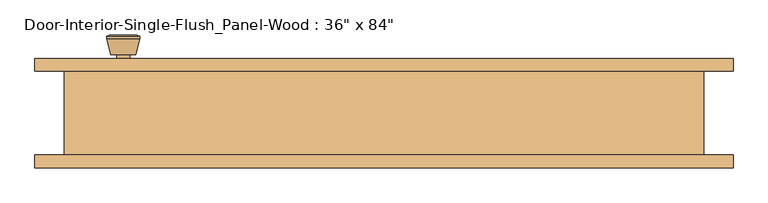
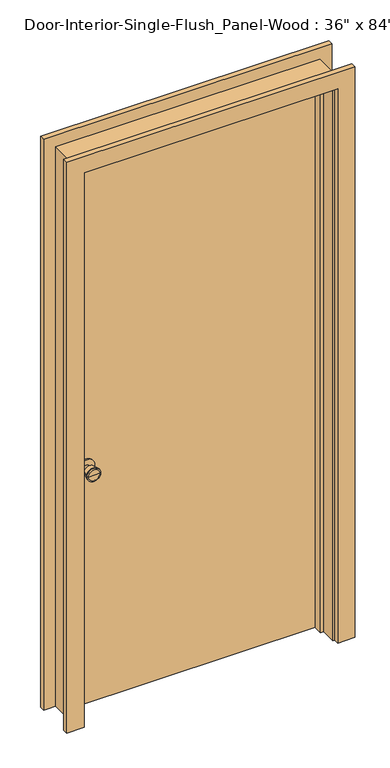
"""IFC4 building model written with IfcOpenShell, lengths in millimetres: door geometry."""

from ifc_helpers import new_model, si_unit, point, frame, frame_2d, origin, origin_with_axes, place, context, project, spatial, polyline, circle_curve, trimmed, segment, composite_curve, outline, extrude, faceted_brep, source, transform, mapped, element, save
from ifc_brep_helpers import plane_surface, cylinder_surface, revolved_surface, advanced_brep


def door_77100466(model_context):
    return source(origin(), model_context, "Body", "SolidModel", [
        advanced_brep(
        [(-393.7, 19.4, 914.4), (-383.7, 19.4, 914.4), (-403.7, 19.4, 914.4), (-373.2241324, -29.6, 914.4), (-393.7, -29.6, 914.4), (-414.1758676, -29.6, 914.4), (-368.7, -27.7721319, 914.4), (-418.7, -27.7721319, 914.4), (-368.7, -24.3084537, 914.4), (-418.7, -24.3084537, 914.4), (-375.063764, 0.4, 914.4), (-412.336236, 0.4, 914.4), (-383.7, 0.4, 914.4), (-403.7, 0.4, 914.4)],
        [
            (0, 1),
            (1, 2, circle_curve(frame((-393.7, 19.4, 914.4), z_axis=(0.0, 1.0, 0.0), x_axis=(-1.0, 0.0, 0.0)), 10.0)),
            (2, 0),
            (2, 1, circle_curve(frame((-393.7, 19.4, 914.4), z_axis=(0.0, 1.0, 0.0), x_axis=(-1.0, 0.0, 0.0)), 10.0)),
            (3, 4),
            (4, 5),
            (5, 3, circle_curve(frame((-393.7, -29.6, 914.4), z_axis=(0.0, -1.0, 0.0), x_axis=(-1.0, 0.0, 0.0)), 20.4758676)),
            (3, 5, circle_curve(frame((-393.7, -29.6, 914.4), z_axis=(0.0, -1.0, 0.0), x_axis=(-1.0, 0.0, 0.0)), 20.4758676)),
            (6, 3),
            (5, 7),
            (7, 6, circle_curve(frame((-393.7, -27.7721319, 914.4), z_axis=(0.0, -1.0, 0.0), x_axis=(-1.0, 0.0, 0.0)), 25.0)),
            (6, 7, circle_curve(frame((-393.7, -27.7721319, 914.4), z_axis=(0.0, -1.0, 0.0), x_axis=(-1.0, 0.0, 0.0)), 25.0)),
            (8, 6),
            (7, 9),
            (9, 8, circle_curve(frame((-393.7, -24.3084537, 914.4), z_axis=(0.0, -1.0, 0.0), x_axis=(-1.0, 0.0, 0.0)), 25.0)),
            (8, 9, circle_curve(frame((-393.7, -24.3084537, 914.4), z_axis=(0.0, -1.0, 0.0), x_axis=(-1.0, 0.0, 0.0)), 25.0)),
            (10, 8),
            (9, 11),
            (11, 10, circle_curve(frame((-393.7, 0.4, 914.4), z_axis=(0.0, -1.0, 0.0), x_axis=(-1.0, 0.0, 0.0)), 18.636236)),
            (10, 11, circle_curve(frame((-393.7, 0.4, 914.4), z_axis=(0.0, -1.0, 0.0), x_axis=(-1.0, 0.0, 0.0)), 18.636236)),
            (12, 10),
            (11, 13),
            (13, 12, circle_curve(frame((-393.7, 0.4, 914.4), z_axis=(0.0, -1.0, 0.0), x_axis=(-1.0, 0.0, 0.0)), 10.0)),
            (12, 13, circle_curve(frame((-393.7, 0.4, 914.4), z_axis=(0.0, -1.0, 0.0), x_axis=(-1.0, 0.0, 0.0)), 10.0)),
            (1, 12),
            (13, 2),
        ],
        [
            plane_surface(frame((-393.7, 19.4, 914.4), z_axis=(0.0, 1.0, 0.0), x_axis=(-1.0, 0.0, 0.0))),
            plane_surface(frame((-393.7, -29.6, 914.4), z_axis=(0.0, -1.0, 0.0), x_axis=(-1.0, 0.0, 0.0))),
            revolved_surface(polyline([(-414.1758676, -29.6, 914.4), (-418.7, -27.7721319, 914.4)]), (-393.7, 19.4, 914.4), (0.0, 1.0, 0.0)),
            cylinder_surface(frame((-393.7, 19.4, 914.4), z_axis=(0.0, 1.0, 0.0), x_axis=(-1.0, 0.0, 0.0)), 25.0),
            revolved_surface(polyline([(-418.7, -24.3084537, 914.4), (-412.336236, 0.4, 914.4)]), (-393.7, 19.4, 914.4), (0.0, 1.0, 0.0)),
            plane_surface(frame((-393.7, 0.4, 914.4), z_axis=(0.0, 1.0, 0.0), x_axis=(-1.0, 0.0, 0.0))),
            cylinder_surface(frame((-393.7, 19.4, 914.4), z_axis=(0.0, 1.0, 0.0), x_axis=(-1.0, 0.0, 0.0)), 10.0),
        ],
        [
            (0, [[1, 2, 3]]),
            (0, [[-3, 4, -1]]),
            (1, [[5, 6, 7]]),
            (1, [[-6, -5, 8]]),
            (2, [[9, -7, 10, 11]]),
            (2, [[-10, -8, -9, 12]]),
            (3, [[13, -11, 14, 15]]),
            (3, [[-14, -12, -13, 16]]),
            (4, [[17, -15, 18, 19]]),
            (4, [[-18, -16, -17, 20]]),
            (5, [[21, -19, 22, 23]]),
            (5, [[-22, -20, -21, 24]]),
            (6, [[25, -23, 26, -2]]),
            (6, [[-26, -24, -25, -4]]),
        ],
    ),
        extrude(outline(composite_curve([segment(trimmed(circle_curve(frame_2d((914.4, -393.7)), 30.0), [point((914.4, -423.7))], [point((914.4, -363.7))], False, "CARTESIAN"), True, "CONTINUOUS"), segment(trimmed(circle_curve(frame_2d((914.4, -393.7)), 30.0), [point((914.4, -363.7))], [point((914.4, -423.7))], False, "CARTESIAN"), True, "CONTINUOUS")], self_intersect=False)), frame((0.0, 19.4, 0.0), z_axis=(0.0, 1.0, 0.0), x_axis=(0.0, 0.0, 1.0)), (0.0, 0.0, 1.0), 6.0),
        advanced_brep(
        [(-393.7, 66.325, 914.4), (-403.7, 66.325, 914.4), (-383.7, 66.325, 914.4), (-373.2241324, 115.325, 914.4), (-414.1758676, 115.325, 914.4), (-393.7, 115.325, 914.4), (-368.7, 113.4971319, 914.4), (-418.7, 113.4971319, 914.4), (-368.7, 110.0334537, 914.4), (-418.7, 110.0334537, 914.4), (-375.063764, 85.325, 914.4), (-412.336236, 85.325, 914.4), (-383.7, 85.325, 914.4), (-403.7, 85.325, 914.4)],
        [
            (0, 1),
            (1, 2, circle_curve(frame((-393.7, 66.325, 914.4), z_axis=(0.0, -1.0, 0.0), x_axis=(-1.0, 0.0, 0.0)), 10.0)),
            (2, 0),
            (2, 1, circle_curve(frame((-393.7, 66.325, 914.4), z_axis=(0.0, -1.0, 0.0), x_axis=(-1.0, 0.0, 0.0)), 10.0)),
            (3, 4, circle_curve(frame((-393.7, 115.325, 914.4), z_axis=(0.0, 1.0, 0.0), x_axis=(-1.0, 0.0, 0.0)), 20.4758676)),
            (4, 5),
            (5, 3),
            (4, 3, circle_curve(frame((-393.7, 115.325, 914.4), z_axis=(0.0, 1.0, 0.0), x_axis=(-1.0, 0.0, 0.0)), 20.4758676)),
            (6, 7, circle_curve(frame((-393.7, 113.4971319, 914.4), z_axis=(0.0, 1.0, 0.0), x_axis=(-1.0, 0.0, 0.0)), 25.0)),
            (7, 4),
            (3, 6),
            (7, 6, circle_curve(frame((-393.7, 113.4971319, 914.4), z_axis=(0.0, 1.0, 0.0), x_axis=(-1.0, 0.0, 0.0)), 25.0)),
            (8, 9, circle_curve(frame((-393.7, 110.0334537, 914.4), z_axis=(0.0, 1.0, 0.0), x_axis=(-1.0, 0.0, 0.0)), 25.0)),
            (9, 7),
            (6, 8),
            (9, 8, circle_curve(frame((-393.7, 110.0334537, 914.4), z_axis=(0.0, 1.0, 0.0), x_axis=(-1.0, 0.0, 0.0)), 25.0)),
            (10, 11, circle_curve(frame((-393.7, 85.325, 914.4), z_axis=(0.0, 1.0, 0.0), x_axis=(-1.0, 0.0, 0.0)), 18.636236)),
            (11, 9),
            (8, 10),
            (11, 10, circle_curve(frame((-393.7, 85.325, 914.4), z_axis=(0.0, 1.0, 0.0), x_axis=(-1.0, 0.0, 0.0)), 18.636236)),
            (12, 13, circle_curve(frame((-393.7, 85.325, 914.4), z_axis=(0.0, 1.0, 0.0), x_axis=(-1.0, 0.0, 0.0)), 10.0)),
            (13, 11),
            (10, 12),
            (13, 12, circle_curve(frame((-393.7, 85.325, 914.4), z_axis=(0.0, 1.0, 0.0), x_axis=(-1.0, 0.0, 0.0)), 10.0)),
            (1, 13),
            (12, 2),
        ],
        [
            plane_surface(frame((-393.7, 66.325, 914.4), z_axis=(0.0, -1.0, 0.0), x_axis=(-1.0, 0.0, 0.0))),
            plane_surface(frame((-393.7, 115.325, 914.4), z_axis=(0.0, 1.0, 0.0), x_axis=(-1.0, 0.0, 0.0))),
            revolved_surface(polyline([(-414.1758676, 115.325, 914.4), (-418.7, 113.4971319, 914.4)]), (-393.7, 66.325, 914.4), (0.0, -1.0, 0.0)),
            cylinder_surface(frame((-393.7, 66.325, 914.4), z_axis=(0.0, -1.0, 0.0), x_axis=(-1.0, 0.0, 0.0)), 25.0),
            revolved_surface(polyline([(-418.7, 110.0334537, 914.4), (-412.336236, 85.325, 914.4)]), (-393.7, 66.325, 914.4), (0.0, -1.0, 0.0)),
            plane_surface(frame((-393.7, 85.325, 914.4), z_axis=(0.0, -1.0, 0.0), x_axis=(-1.0, 0.0, 0.0))),
            cylinder_surface(frame((-393.7, 66.325, 914.4), z_axis=(0.0, -1.0, 0.0), x_axis=(-1.0, 0.0, 0.0)), 10.0),
        ],
        [
            (0, [[1, 2, 3]]),
            (0, [[-3, 4, -1]]),
            (1, [[5, 6, 7]]),
            (1, [[8, -7, -6]]),
            (2, [[9, 10, -5, 11]]),
            (2, [[12, -11, -8, -10]]),
            (3, [[13, 14, -9, 15]]),
            (3, [[16, -15, -12, -14]]),
            (4, [[17, 18, -13, 19]]),
            (4, [[20, -19, -16, -18]]),
            (5, [[21, 22, -17, 23]]),
            (5, [[24, -23, -20, -22]]),
            (6, [[-2, 25, -21, 26]]),
            (6, [[-4, -26, -24, -25]]),
        ],
    ),
        extrude(outline(composite_curve([segment(trimmed(circle_curve(frame_2d((914.4, -393.7)), 30.0), [point((914.4, -423.7))], [point((914.4, -363.7))], False, "CARTESIAN"), True, "CONTINUOUS"), segment(trimmed(circle_curve(frame_2d((914.4, -393.7)), 30.0), [point((914.4, -363.7))], [point((914.4, -423.7))], False, "CARTESIAN"), True, "CONTINUOUS")], self_intersect=False)), frame((0.0, 60.325, 0.0), z_axis=(0.0, 1.0, 0.0), x_axis=(0.0, 0.0, 1.0)), (0.0, 0.0, 1.0), 6.0),
        extrude(outline(polyline([(457.2, 25.4), (-457.2, 25.4), (-457.2, 60.325), (457.2, 60.325), (457.2, 25.4)])), origin_with_axes(), (0.0, 0.0, 1.0), 2133.6),
        faceted_brep([(482.6, 60.325, 0.0), (482.6, -66.675, 0.0), (457.2, -66.675, 0.0), (457.2, -9.525, 0.0), (444.5, -9.525, 0.0), (444.5, 25.4, 0.0), (457.2, 25.4, 0.0), (457.2, 60.325, 0.0), (482.6, 60.325, 2159.0), (482.6, -66.675, 2159.0), (-482.6, -66.675, 2159.0), (-482.6, -66.675, 0.0), (-457.2, -66.675, 0.0), (-457.2, -66.675, 2133.6), (457.2, -66.675, 2133.6), (457.2, -9.525, 2133.6), (-457.2, -9.525, 2133.6), (-457.2, -9.525, 0.0), (-444.5, -9.525, 0.0), (-444.5, -9.525, 2120.9), (444.5, -9.525, 2120.9), (444.5, 25.4, 2120.9), (-444.5, 25.4, 2120.9), (-444.5, 25.4, 0.0), (-457.2, 25.4, 0.0), (-457.2, 25.4, 2133.6), (457.2, 25.4, 2133.6), (457.2, 60.325, 2133.6), (-457.2, 60.325, 2133.6), (-457.2, 60.325, 0.0), (-482.6, 60.325, 0.0), (-482.6, 60.325, 2159.0)], [[[0, 1, 2, 3, 4, 5, 6, 7]], [[1, 0, 8, 9]], [[2, 1, 9, 10, 11, 12, 13, 14]], [[3, 2, 14, 15]], [[4, 3, 15, 16, 17, 18, 19, 20]], [[5, 4, 20, 21]], [[6, 5, 21, 22, 23, 24, 25, 26]], [[7, 6, 26, 27]], [[0, 7, 27, 28, 29, 30, 31, 8]], [[9, 8, 31, 10]], [[15, 14, 13, 16]], [[21, 20, 19, 22]], [[27, 26, 25, 28]], [[30, 29, 24, 23, 18, 17, 12, 11]], [[10, 31, 30, 11]], [[16, 13, 12, 17]], [[22, 19, 18, 23]], [[28, 25, 24, 29]]]),
        extrude(outline(polyline([(0.0, 463.55), (0.0, 527.05), (2203.45, 527.05), (2203.45, -527.05), (0.0, -527.05), (0.0, -463.55), (2139.95, -463.55), (2139.95, 463.55), (0.0, 463.55)])), frame((0.0, -85.725, 0.0), z_axis=(0.0, 1.0, 0.0), x_axis=(0.0, 0.0, 1.0)), (0.0, 0.0, 1.0), 19.05),
        extrude(outline(polyline([(0.0, 463.55), (0.0, 527.05), (2203.45, 527.05), (2203.45, -527.05), (0.0, -527.05), (0.0, -463.55), (2139.95, -463.55), (2139.95, 463.55), (0.0, 463.55)])), frame((0.0, 60.325, 0.0), z_axis=(0.0, 1.0, 0.0), x_axis=(0.0, 0.0, 1.0)), (0.0, 0.0, 1.0), 19.05),
    ])


if __name__ == "__main__":
    model = new_model("IFC4")
    model_context = context("Model", 3, world=origin())
    ifc_project = project(units=[si_unit("LENGTHUNIT", "METRE", prefix="MILLI")], contexts=[model_context])
    site = spatial("IfcSite", under=ifc_project)
    building = spatial("IfcBuilding", under=site)
    placement = place(None, origin())
    door_shape = door_77100466(model_context)
    element("IfcDoor", 1, ObjectType="Door-Interior-Single-Flush_Panel-Wood : 36\" x 84\"", at=placement, inside=building, context=model_context, shape_type="MappedRepresentation", body=[
        mapped(door_shape, transform((0.0, 0.0, 0.0), x_axis=(1.0, 0.0, 0.0), y_axis=(0.0, 1.0, 0.0), z_axis=(0.0, 0.0, 1.0))),
    ])
    save(model, "model.ifc")

# Revit data of these elements
# Type "Door-Interior-Single-Flush_Panel-Wood : 36\" x 84\""
#   Type Mark = "2"
#   Assembly Code = "C1020300"
#   Analytic Construction = "Wooden"
#   Thickness = 0' - 1 3/8"
#   Thermal Resistance (R) = 0.455703 (m²·K)/W
#   Swing Angle [instance default] = 90.00°
#   Rough Width = 3' - 2"
#   Rough Height = 7' - 1"
#   Height = 7' - 0"
#   Width = 3' - 0"
#   Heat Transfer Coefficient (U) = 2.19465 W/(m²·K)
#   Trim Material = Cherry
#   Panel Material = Cherry
#   Frame Material = Cherry
#   Door Handle Material = Aluminum
#   Visual Light Transmittance = 0
#   Solar Heat Gain Coefficient = 0
#   Wall Closure = (empty or 0)
#   Function = (empty or 0)
# Element 1 (IfcDoor, "Door-Interior-Single-Flush_Panel-Wood : 36\" x 84\"")
#   Materials on its faces: "Cherry", "Aluminum"
# Materials
#   "Cherry": class "Wood", colour RGB 154 107 61, transparency 0, Description = "Prunus Serotina", Cost = 0
#   "Aluminum": class "Metal", colour RGB 244 244 244, transparency 0, Description = "Aluminum 6061", Cost = 0
